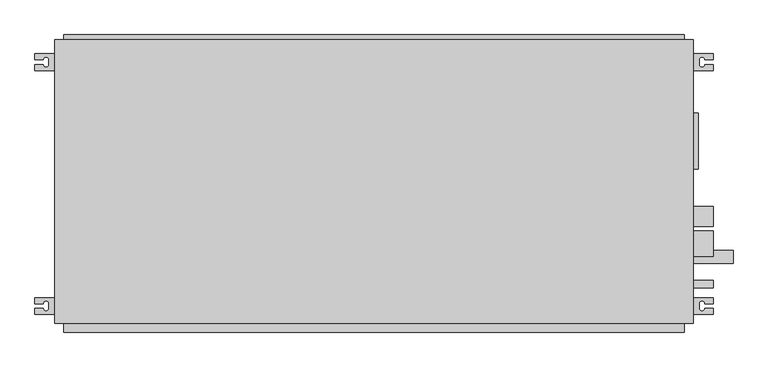
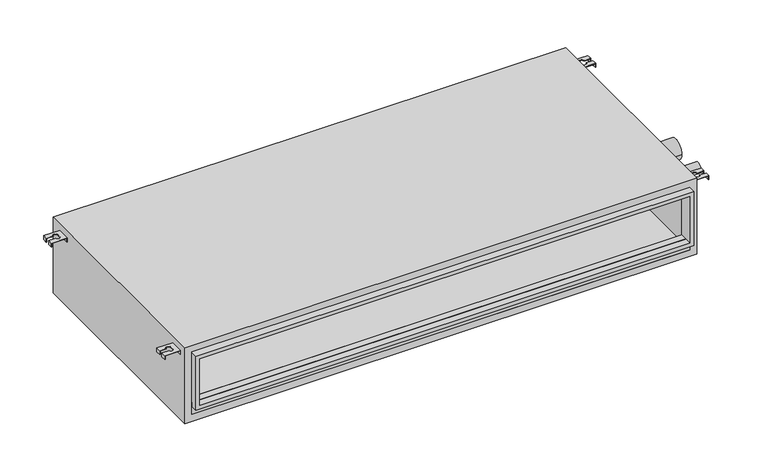
"""IFC4 building model written with IfcOpenShell, lengths in millimetres: proxy geometry, PEFY-P-NMAU-E_Medium_Static_Ducted : PEFY-P54NMAU-E."""

from ifc_helpers import new_model, si_unit, point, frame, frame_2d, origin, place, context, project, spatial, polyline, circle_curve, trimmed, segment, composite_curve, outline, extrude, source, transform, mapped, element, save
from ifc_brep_helpers import plane_surface, revolved_surface, advanced_brep


def mechanical_equipment_8a2286fb(model_context):
    return source(origin(), model_context, "Body", "SolidModel", [
        advanced_brep(
        [(-860.118493, -231.05, 249.2375), (-860.118493, -246.05, 249.2375), (-839.112243, -246.05, 249.2375), (-825.112243, -246.05, 249.2375), (-825.112243, -258.05, 249.2375), (-839.112243, -258.05, 249.2375), (-860.118493, -258.05, 249.2375), (-860.118493, -273.05, 249.2375), (-810.112243, -273.05, 249.2375), (-810.112243, -231.05, 249.2375), (-860.118493, -231.05, 236.4972162), (-858.530493, -231.05, 236.4972162), (-858.530493, -246.05, 236.4972162), (-860.118493, -246.05, 236.4972162), (-858.530493, -273.05, 236.4972162), (-860.118493, -273.05, 236.4972162), (-860.118493, -258.05, 236.4972162), (-858.530493, -258.05, 236.4972162), (-810.112243, -231.05, 236.4972162), (-810.112243, -273.05, 236.4972162), (-811.700243, -273.05, 236.4972162), (-811.700243, -231.05, 236.4972162), (-858.530493, -246.05, 247.65), (-839.112243, -246.05, 247.65), (-858.530493, -231.05, 247.65), (-811.700243, -231.05, 247.65), (-858.530493, -258.05, 247.65), (-858.530493, -273.05, 247.65), (-839.112243, -258.05, 247.65), (-811.700243, -273.05, 247.65), (-825.112243, -258.05, 247.65), (-825.112243, -246.05, 247.65)],
        [
            (0, 1),
            (1, 2),
            (2, 3, circle_curve(frame((-832.112243, -246.05, 249.2375), z_axis=(0.0, 0.0, -1.0), x_axis=(1.0, 0.0, 0.0)), 7.0)),
            (3, 4),
            (4, 5, circle_curve(frame((-832.112243, -258.05, 249.2375), z_axis=(0.0, 0.0, -1.0), x_axis=(1.0, 0.0, 0.0)), 7.0)),
            (5, 6),
            (6, 7),
            (7, 8),
            (8, 9),
            (9, 0),
            (10, 11),
            (11, 12),
            (12, 13),
            (13, 10),
            (14, 15),
            (15, 16),
            (16, 17),
            (17, 14),
            (18, 19),
            (19, 20),
            (20, 21),
            (21, 18),
            (13, 1),
            (0, 10),
            (12, 22),
            (22, 23),
            (23, 2),
            (11, 24),
            (24, 22),
            (9, 18),
            (21, 25),
            (25, 24),
            (17, 26),
            (26, 27),
            (27, 14),
            (5, 28),
            (28, 26),
            (16, 6),
            (15, 7),
            (27, 29),
            (29, 20),
            (19, 8),
            (29, 25),
            (30, 31),
            (31, 23, circle_curve(frame((-832.112243, -246.05, 247.65), z_axis=(0.0, 0.0, 1.0), x_axis=(1.0, 0.0, 0.0)), 7.0)),
            (28, 30, circle_curve(frame((-832.112243, -258.05, 247.65), z_axis=(0.0, 0.0, 1.0), x_axis=(1.0, 0.0, 0.0)), 7.0)),
            (4, 30),
            (31, 3),
        ],
        [
            plane_surface(frame((-860.118493, -231.05, 249.2375), z_axis=(0.0, 0.0, 1.0), x_axis=(0.0, -1.0, 0.0))),
            plane_surface(frame((-860.118493, -231.05, 236.4972162), z_axis=(0.0, 0.0, -1.0), x_axis=(0.0, 1.0, 0.0))),
            plane_surface(frame((-860.118493, -231.05, 249.2375), z_axis=(-1.0, 0.0, 0.0), x_axis=(0.0, 0.0, -1.0))),
            plane_surface(frame((-860.118493, -246.05, 249.2375), z_axis=(0.0, -1.0, 0.0), x_axis=(0.0, 0.0, -1.0))),
            plane_surface(frame((-858.530493, -246.05, 249.2375), z_axis=(1.0, 0.0, 0.0), x_axis=(0.0, 0.0, -1.0))),
            plane_surface(frame((-858.530493, -231.05, 249.2375), z_axis=(0.0, 1.0, 0.0), x_axis=(0.0, 0.0, -1.0))),
            plane_surface(frame((-858.530493, -273.05, 249.2375), z_axis=(1.0, 0.0, 0.0), x_axis=(0.0, 0.0, -1.0))),
            plane_surface(frame((-858.530493, -258.05, 249.2375), z_axis=(0.0, 1.0, 0.0), x_axis=(0.0, 0.0, -1.0))),
            plane_surface(frame((-860.118493, -258.05, 249.2375), z_axis=(-1.0, 0.0, 0.0), x_axis=(0.0, 0.0, -1.0))),
            plane_surface(frame((-860.118493, -273.05, 249.2375), z_axis=(0.0, -1.0, 0.0), x_axis=(0.0, 0.0, -1.0))),
            plane_surface(frame((-811.700243, -231.05, 249.2375), z_axis=(-1.0, 0.0, 0.0), x_axis=(0.0, 0.0, -1.0))),
            plane_surface(frame((-810.112243, -273.05, 249.2375), z_axis=(1.0, 0.0, 0.0), x_axis=(0.0, 0.0, -1.0))),
            plane_surface(frame((-825.112243, -258.05, 247.65), z_axis=(0.0, 0.0, -1.0), x_axis=(0.0, 1.0, 0.0))),
            revolved_surface(polyline([(-825.112243, -258.05, 247.65), (-825.112243, -258.05, 249.2375)]), (-832.112243, -258.05, 247.65), (0.0, 0.0, -1.0)),
            revolved_surface(polyline([(-825.112243, -246.05, 247.65), (-825.112243, -246.05, 249.2375)]), (-832.112243, -246.05, 247.65), (0.0, 0.0, -1.0)),
            plane_surface(frame((-825.112243, -246.05, 249.2375), z_axis=(-1.0, 0.0, 0.0), x_axis=(0.0, 0.0, -1.0))),
        ],
        [
            (0, [[1, 2, 3, 4, 5, 6, 7, 8, 9, 10]]),
            (1, [[11, 12, 13, 14]]),
            (1, [[15, 16, 17, 18]]),
            (1, [[19, 20, 21, 22]]),
            (2, [[23, -1, 24, -14]]),
            (3, [[-2, -23, -13, 25, 26, 27]]),
            (4, [[-12, 28, 29, -25]]),
            (5, [[-10, 30, -22, 31, 32, -28, -11, -24]]),
            (6, [[-18, 33, 34, 35]]),
            (7, [[-6, 36, 37, -33, -17, 38]]),
            (8, [[39, -7, -38, -16]]),
            (9, [[-8, -39, -15, -35, 40, 41, -20, 42]]),
            (10, [[-21, -41, 43, -31]]),
            (11, [[-30, -9, -42, -19]]),
            (12, [[44, 45, -26, -29, -32, -43, -40, -34, -37, 46]]),
            (13, [[-5, 47, -46, -36]]),
            (14, [[-3, -27, -45, 48]]),
            (15, [[-4, -48, -44, -47]]),
        ],
    ),
        advanced_brep(
        [(840.094007, -231.05, 249.2375), (790.087757, -231.05, 249.2375), (790.087757, -273.05, 249.2375), (840.094007, -273.05, 249.2375), (840.094007, -258.05, 249.2375), (819.087757, -258.05, 249.2375), (805.087757, -258.05, 249.2375), (805.087757, -246.05, 249.2375), (819.087757, -246.05, 249.2375), (840.094007, -246.05, 249.2375), (840.094007, -231.05, 236.4972162), (840.094007, -246.05, 236.4972162), (838.506007, -246.05, 236.4972162), (838.506007, -231.05, 236.4972162), (838.506007, -273.05, 236.4972162), (838.506007, -258.05, 236.4972162), (840.094007, -258.05, 236.4972162), (840.094007, -273.05, 236.4972162), (790.087757, -231.05, 236.4972162), (791.675757, -231.05, 236.4972162), (791.675757, -273.05, 236.4972162), (790.087757, -273.05, 236.4972162), (819.087757, -246.05, 247.65), (838.506007, -246.05, 247.65), (838.506007, -231.05, 247.65), (791.675757, -231.05, 247.65), (838.506007, -273.05, 247.65), (838.506007, -258.05, 247.65), (819.087757, -258.05, 247.65), (791.675757, -273.05, 247.65), (805.087757, -258.05, 247.65), (805.087757, -246.05, 247.65)],
        [
            (0, 1),
            (1, 2),
            (2, 3),
            (3, 4),
            (4, 5),
            (5, 6, circle_curve(frame((812.087757, -258.05, 249.2375), z_axis=(0.0, 0.0, -1.0), x_axis=(-1.0, 0.0, 0.0)), 7.0)),
            (6, 7),
            (7, 8, circle_curve(frame((812.087757, -246.05, 249.2375), z_axis=(0.0, 0.0, -1.0), x_axis=(-1.0, 0.0, 0.0)), 7.0)),
            (8, 9),
            (9, 0),
            (10, 11),
            (11, 12),
            (12, 13),
            (13, 10),
            (14, 15),
            (15, 16),
            (16, 17),
            (17, 14),
            (18, 19),
            (19, 20),
            (20, 21),
            (21, 18),
            (10, 0),
            (9, 11),
            (8, 22),
            (22, 23),
            (23, 12),
            (23, 24),
            (24, 13),
            (24, 25),
            (25, 19),
            (18, 1),
            (14, 26),
            (26, 27),
            (27, 15),
            (4, 16),
            (27, 28),
            (28, 5),
            (3, 17),
            (2, 21),
            (20, 29),
            (29, 26),
            (25, 29),
            (30, 28, circle_curve(frame((812.087757, -258.05, 247.65), z_axis=(0.0, 0.0, 1.0), x_axis=(-1.0, 0.0, 0.0)), 7.0)),
            (22, 31, circle_curve(frame((812.087757, -246.05, 247.65), z_axis=(0.0, 0.0, 1.0), x_axis=(-1.0, 0.0, 0.0)), 7.0)),
            (31, 30),
            (30, 6),
            (7, 31),
        ],
        [
            plane_surface(frame((840.094007, -231.05, 249.2375), z_axis=(0.0, 0.0, 1.0), x_axis=(0.0, -1.0, 0.0))),
            plane_surface(frame((840.094007, -231.05, 236.4972162), z_axis=(0.0, 0.0, -1.0), x_axis=(0.0, 1.0, 0.0))),
            plane_surface(frame((840.094007, -231.05, 249.2375), z_axis=(1.0, 0.0, 0.0), x_axis=(0.0, 0.0, -1.0))),
            plane_surface(frame((840.094007, -246.05, 249.2375), z_axis=(0.0, -1.0, 0.0), x_axis=(0.0, 0.0, -1.0))),
            plane_surface(frame((838.506007, -246.05, 249.2375), z_axis=(-1.0, 0.0, 0.0), x_axis=(0.0, 0.0, -1.0))),
            plane_surface(frame((838.506007, -231.05, 249.2375), z_axis=(0.0, 1.0, 0.0), x_axis=(0.0, 0.0, -1.0))),
            plane_surface(frame((838.506007, -273.05, 249.2375), z_axis=(-1.0, 0.0, 0.0), x_axis=(0.0, 0.0, -1.0))),
            plane_surface(frame((838.506007, -258.05, 249.2375), z_axis=(0.0, 1.0, 0.0), x_axis=(0.0, 0.0, -1.0))),
            plane_surface(frame((840.094007, -258.05, 249.2375), z_axis=(1.0, 0.0, 0.0), x_axis=(0.0, 0.0, -1.0))),
            plane_surface(frame((840.094007, -273.05, 249.2375), z_axis=(0.0, -1.0, 0.0), x_axis=(0.0, 0.0, -1.0))),
            plane_surface(frame((791.675757, -231.05, 249.2375), z_axis=(1.0, 0.0, 0.0), x_axis=(0.0, 0.0, -1.0))),
            plane_surface(frame((790.087757, -273.05, 249.2375), z_axis=(-1.0, 0.0, 0.0), x_axis=(0.0, 0.0, -1.0))),
            plane_surface(frame((805.087757, -258.05, 247.65), z_axis=(0.0, 0.0, -1.0), x_axis=(0.0, 1.0, 0.0))),
            revolved_surface(polyline([(805.087757, -258.05, 247.65), (805.087757, -258.05, 249.2375)]), (812.087757, -258.05, 247.65), (0.0, 0.0, -1.0)),
            revolved_surface(polyline([(805.087757, -246.05, 247.65), (805.087757, -246.05, 249.2375)]), (812.087757, -246.05, 247.65), (0.0, 0.0, -1.0)),
            plane_surface(frame((805.087757, -246.05, 249.2375), z_axis=(1.0, 0.0, 0.0), x_axis=(0.0, 0.0, -1.0))),
        ],
        [
            (0, [[1, 2, 3, 4, 5, 6, 7, 8, 9, 10]]),
            (1, [[11, 12, 13, 14]]),
            (1, [[15, 16, 17, 18]]),
            (1, [[19, 20, 21, 22]]),
            (2, [[-11, 23, -10, 24]]),
            (3, [[25, 26, 27, -12, -24, -9]]),
            (4, [[-27, 28, 29, -13]]),
            (5, [[-23, -14, -29, 30, 31, -19, 32, -1]]),
            (6, [[33, 34, 35, -15]]),
            (7, [[36, -16, -35, 37, 38, -5]]),
            (8, [[-17, -36, -4, 39]]),
            (9, [[40, -21, 41, 42, -33, -18, -39, -3]]),
            (10, [[-31, 43, -41, -20]]),
            (11, [[-22, -40, -2, -32]]),
            (12, [[44, -37, -34, -42, -43, -30, -28, -26, 45, 46]]),
            (13, [[-38, -44, 47, -6]]),
            (14, [[48, -45, -25, -8]]),
            (15, [[-47, -46, -48, -7]]),
        ],
    ),
        advanced_brep(
        [(-860.118493, 339.0, 249.2375), (-810.112243, 339.0, 249.2375), (-810.112243, 381.0, 249.2375), (-860.118493, 381.0, 249.2375), (-860.118493, 366.0, 249.2375), (-839.112243, 366.0, 249.2375), (-825.112243, 366.0, 249.2375), (-825.112243, 354.0, 249.2375), (-839.112243, 354.0, 249.2375), (-860.118493, 354.0, 249.2375), (-860.118493, 339.0, 236.4972162), (-860.118493, 354.0, 236.4972162), (-858.530493, 354.0, 236.4972162), (-858.530493, 339.0, 236.4972162), (-858.530493, 381.0, 236.4972162), (-858.530493, 366.0, 236.4972162), (-860.118493, 366.0, 236.4972162), (-860.118493, 381.0, 236.4972162), (-810.112243, 339.0, 236.4972162), (-811.700243, 339.0, 236.4972162), (-811.700243, 381.0, 236.4972162), (-810.112243, 381.0, 236.4972162), (-839.112243, 354.0, 247.65), (-858.530493, 354.0, 247.65), (-858.530493, 339.0, 247.65), (-811.700243, 339.0, 247.65), (-858.530493, 381.0, 247.65), (-858.530493, 366.0, 247.65), (-839.112243, 366.0, 247.65), (-811.700243, 381.0, 247.65), (-825.112243, 366.0, 247.65), (-825.112243, 354.0, 247.65)],
        [
            (0, 1),
            (1, 2),
            (2, 3),
            (3, 4),
            (4, 5),
            (5, 6, circle_curve(frame((-832.112243, 366.0, 249.2375), z_axis=(0.0, 0.0, -1.0), x_axis=(1.0, 0.0, 0.0)), 7.0)),
            (6, 7),
            (7, 8, circle_curve(frame((-832.112243, 354.0, 249.2375), z_axis=(0.0, 0.0, -1.0), x_axis=(1.0, 0.0, 0.0)), 7.0)),
            (8, 9),
            (9, 0),
            (10, 11),
            (11, 12),
            (12, 13),
            (13, 10),
            (14, 15),
            (15, 16),
            (16, 17),
            (17, 14),
            (18, 19),
            (19, 20),
            (20, 21),
            (21, 18),
            (10, 0),
            (9, 11),
            (8, 22),
            (22, 23),
            (23, 12),
            (23, 24),
            (24, 13),
            (24, 25),
            (25, 19),
            (18, 1),
            (14, 26),
            (26, 27),
            (27, 15),
            (4, 16),
            (27, 28),
            (28, 5),
            (3, 17),
            (2, 21),
            (20, 29),
            (29, 26),
            (25, 29),
            (30, 28, circle_curve(frame((-832.112243, 366.0, 247.65), z_axis=(0.0, 0.0, 1.0), x_axis=(1.0, 0.0, 0.0)), 7.0)),
            (22, 31, circle_curve(frame((-832.112243, 354.0, 247.65), z_axis=(0.0, 0.0, 1.0), x_axis=(1.0, 0.0, 0.0)), 7.0)),
            (31, 30),
            (30, 6),
            (7, 31),
        ],
        [
            plane_surface(frame((-860.118493, 339.0, 249.2375), z_axis=(0.0, 0.0, 1.0), x_axis=(0.0, 1.0, 0.0))),
            plane_surface(frame((-860.118493, 339.0, 236.4972162), z_axis=(0.0, 0.0, -1.0), x_axis=(0.0, -1.0, 0.0))),
            plane_surface(frame((-860.118493, 339.0, 249.2375), z_axis=(-1.0, 0.0, 0.0), x_axis=(0.0, 0.0, -1.0))),
            plane_surface(frame((-860.118493, 354.0, 249.2375), z_axis=(0.0, 1.0, 0.0), x_axis=(0.0, 0.0, -1.0))),
            plane_surface(frame((-858.530493, 354.0, 249.2375), z_axis=(1.0, 0.0, 0.0), x_axis=(0.0, 0.0, -1.0))),
            plane_surface(frame((-858.530493, 339.0, 249.2375), z_axis=(0.0, -1.0, 0.0), x_axis=(0.0, 0.0, -1.0))),
            plane_surface(frame((-858.530493, 381.0, 249.2375), z_axis=(1.0, 0.0, 0.0), x_axis=(0.0, 0.0, -1.0))),
            plane_surface(frame((-858.530493, 366.0, 249.2375), z_axis=(0.0, -1.0, 0.0), x_axis=(0.0, 0.0, -1.0))),
            plane_surface(frame((-860.118493, 366.0, 249.2375), z_axis=(-1.0, 0.0, 0.0), x_axis=(0.0, 0.0, -1.0))),
            plane_surface(frame((-860.118493, 381.0, 249.2375), z_axis=(0.0, 1.0, 0.0), x_axis=(0.0, 0.0, -1.0))),
            plane_surface(frame((-811.700243, 339.0, 249.2375), z_axis=(-1.0, 0.0, 0.0), x_axis=(0.0, 0.0, -1.0))),
            plane_surface(frame((-810.112243, 381.0, 249.2375), z_axis=(1.0, 0.0, 0.0), x_axis=(0.0, 0.0, -1.0))),
            plane_surface(frame((-825.112243, 366.0, 247.65), z_axis=(0.0, 0.0, -1.0), x_axis=(0.0, -1.0, 0.0))),
            revolved_surface(polyline([(-825.112243, 366.0, 247.65), (-825.112243, 366.0, 249.2375)]), (-832.112243, 366.0, 247.65), (0.0, 0.0, -1.0)),
            revolved_surface(polyline([(-825.112243, 354.0, 247.65), (-825.112243, 354.0, 249.2375)]), (-832.112243, 354.0, 247.65), (0.0, 0.0, -1.0)),
            plane_surface(frame((-825.112243, 354.0, 249.2375), z_axis=(-1.0, 0.0, 0.0), x_axis=(0.0, 0.0, -1.0))),
        ],
        [
            (0, [[1, 2, 3, 4, 5, 6, 7, 8, 9, 10]]),
            (1, [[11, 12, 13, 14]]),
            (1, [[15, 16, 17, 18]]),
            (1, [[19, 20, 21, 22]]),
            (2, [[-11, 23, -10, 24]]),
            (3, [[25, 26, 27, -12, -24, -9]]),
            (4, [[-27, 28, 29, -13]]),
            (5, [[-23, -14, -29, 30, 31, -19, 32, -1]]),
            (6, [[33, 34, 35, -15]]),
            (7, [[36, -16, -35, 37, 38, -5]]),
            (8, [[-17, -36, -4, 39]]),
            (9, [[40, -21, 41, 42, -33, -18, -39, -3]]),
            (10, [[-31, 43, -41, -20]]),
            (11, [[-22, -40, -2, -32]]),
            (12, [[44, -37, -34, -42, -43, -30, -28, -26, 45, 46]]),
            (13, [[-38, -44, 47, -6]]),
            (14, [[48, -45, -25, -8]]),
            (15, [[-47, -46, -48, -7]]),
        ],
    ),
        advanced_brep(
        [(840.094007, 339.0, 249.2375), (840.094007, 354.0, 249.2375), (819.087757, 354.0, 249.2375), (805.087757, 354.0, 249.2375), (805.087757, 366.0, 249.2375), (819.087757, 366.0, 249.2375), (840.094007, 366.0, 249.2375), (840.094007, 381.0, 249.2375), (790.087757, 381.0, 249.2375), (790.087757, 339.0, 249.2375), (840.094007, 339.0, 236.4972162), (838.506007, 339.0, 236.4972162), (838.506007, 354.0, 236.4972162), (840.094007, 354.0, 236.4972162), (838.506007, 381.0, 236.4972162), (840.094007, 381.0, 236.4972162), (840.094007, 366.0, 236.4972162), (838.506007, 366.0, 236.4972162), (790.087757, 339.0, 236.4972162), (790.087757, 381.0, 236.4972162), (791.675757, 381.0, 236.4972162), (791.675757, 339.0, 236.4972162), (838.506007, 354.0, 247.65), (819.087757, 354.0, 247.65), (838.506007, 339.0, 247.65), (791.675757, 339.0, 247.65), (838.506007, 366.0, 247.65), (838.506007, 381.0, 247.65), (819.087757, 366.0, 247.65), (791.675757, 381.0, 247.65), (805.087757, 366.0, 247.65), (805.087757, 354.0, 247.65)],
        [
            (0, 1),
            (1, 2),
            (2, 3, circle_curve(frame((812.087757, 354.0, 249.2375), z_axis=(0.0, 0.0, -1.0), x_axis=(-1.0, 0.0, 0.0)), 7.0)),
            (3, 4),
            (4, 5, circle_curve(frame((812.087757, 366.0, 249.2375), z_axis=(0.0, 0.0, -1.0), x_axis=(-1.0, 0.0, 0.0)), 7.0)),
            (5, 6),
            (6, 7),
            (7, 8),
            (8, 9),
            (9, 0),
            (10, 11),
            (11, 12),
            (12, 13),
            (13, 10),
            (14, 15),
            (15, 16),
            (16, 17),
            (17, 14),
            (18, 19),
            (19, 20),
            (20, 21),
            (21, 18),
            (13, 1),
            (0, 10),
            (12, 22),
            (22, 23),
            (23, 2),
            (11, 24),
            (24, 22),
            (9, 18),
            (21, 25),
            (25, 24),
            (17, 26),
            (26, 27),
            (27, 14),
            (5, 28),
            (28, 26),
            (16, 6),
            (15, 7),
            (27, 29),
            (29, 20),
            (19, 8),
            (29, 25),
            (30, 31),
            (31, 23, circle_curve(frame((812.087757, 354.0, 247.65), z_axis=(0.0, 0.0, 1.0), x_axis=(-1.0, 0.0, 0.0)), 7.0)),
            (28, 30, circle_curve(frame((812.087757, 366.0, 247.65), z_axis=(0.0, 0.0, 1.0), x_axis=(-1.0, 0.0, 0.0)), 7.0)),
            (4, 30),
            (31, 3),
        ],
        [
            plane_surface(frame((840.094007, 339.0, 249.2375), z_axis=(0.0, 0.0, 1.0), x_axis=(0.0, 1.0, 0.0))),
            plane_surface(frame((840.094007, 339.0, 236.4972162), z_axis=(0.0, 0.0, -1.0), x_axis=(0.0, -1.0, 0.0))),
            plane_surface(frame((840.094007, 339.0, 249.2375), z_axis=(1.0, 0.0, 0.0), x_axis=(0.0, 0.0, -1.0))),
            plane_surface(frame((840.094007, 354.0, 249.2375), z_axis=(0.0, 1.0, 0.0), x_axis=(0.0, 0.0, -1.0))),
            plane_surface(frame((838.506007, 354.0, 249.2375), z_axis=(-1.0, 0.0, 0.0), x_axis=(0.0, 0.0, -1.0))),
            plane_surface(frame((838.506007, 339.0, 249.2375), z_axis=(0.0, -1.0, 0.0), x_axis=(0.0, 0.0, -1.0))),
            plane_surface(frame((838.506007, 381.0, 249.2375), z_axis=(-1.0, 0.0, 0.0), x_axis=(0.0, 0.0, -1.0))),
            plane_surface(frame((838.506007, 366.0, 249.2375), z_axis=(0.0, -1.0, 0.0), x_axis=(0.0, 0.0, -1.0))),
            plane_surface(frame((840.094007, 366.0, 249.2375), z_axis=(1.0, 0.0, 0.0), x_axis=(0.0, 0.0, -1.0))),
            plane_surface(frame((840.094007, 381.0, 249.2375), z_axis=(0.0, 1.0, 0.0), x_axis=(0.0, 0.0, -1.0))),
            plane_surface(frame((791.675757, 339.0, 249.2375), z_axis=(1.0, 0.0, 0.0), x_axis=(0.0, 0.0, -1.0))),
            plane_surface(frame((790.087757, 381.0, 249.2375), z_axis=(-1.0, 0.0, 0.0), x_axis=(0.0, 0.0, -1.0))),
            plane_surface(frame((805.087757, 366.0, 247.65), z_axis=(0.0, 0.0, -1.0), x_axis=(0.0, -1.0, 0.0))),
            revolved_surface(polyline([(805.087757, 366.0, 247.65), (805.087757, 366.0, 249.2375)]), (812.087757, 366.0, 247.65), (0.0, 0.0, -1.0)),
            revolved_surface(polyline([(805.087757, 354.0, 247.65), (805.087757, 354.0, 249.2375)]), (812.087757, 354.0, 247.65), (0.0, 0.0, -1.0)),
            plane_surface(frame((805.087757, 354.0, 249.2375), z_axis=(1.0, 0.0, 0.0), x_axis=(0.0, 0.0, -1.0))),
        ],
        [
            (0, [[1, 2, 3, 4, 5, 6, 7, 8, 9, 10]]),
            (1, [[11, 12, 13, 14]]),
            (1, [[15, 16, 17, 18]]),
            (1, [[19, 20, 21, 22]]),
            (2, [[23, -1, 24, -14]]),
            (3, [[-2, -23, -13, 25, 26, 27]]),
            (4, [[-12, 28, 29, -25]]),
            (5, [[-10, 30, -22, 31, 32, -28, -11, -24]]),
            (6, [[-18, 33, 34, 35]]),
            (7, [[-6, 36, 37, -33, -17, 38]]),
            (8, [[39, -7, -38, -16]]),
            (9, [[-8, -39, -15, -35, 40, 41, -20, 42]]),
            (10, [[-21, -41, 43, -31]]),
            (11, [[-30, -9, -42, -19]]),
            (12, [[44, 45, -26, -29, -32, -43, -40, -34, -37, 46]]),
            (13, [[-5, 47, -46, -36]]),
            (14, [[-3, -27, -45, 48]]),
            (15, [[-4, -48, -44, -47]]),
        ],
    ),
        extrude(outline(polyline([(767.862757, -295.275), (-787.887243, -295.275), (-787.887243, -273.05), (767.862757, -273.05), (767.862757, -295.275)])), frame((0.0, 0.0, 42.8625), z_axis=(0.0, 0.0, 1.0), x_axis=(1.0, 0.0, 0.0)), (0.0, 0.0, 1.0), 39.6875),
        extrude(outline(polyline([(249.2375, 767.862757), (249.2375, -787.887243), (69.85, -787.887243), (69.85, 767.862757), (249.2375, 767.862757)]), holes=[polyline([(82.55, 755.162757), (82.55, -775.187243), (236.5375, -775.187243), (236.5375, 755.162757), (82.55, 755.162757)])]), frame((0.0, -317.5, 0.0), z_axis=(0.0, 1.0, 0.0), x_axis=(0.0, 0.0, 1.0)), (0.0, 0.0, 1.0), 44.45),
        extrude(outline(polyline([(767.862757, 415.925), (-787.887243, 415.925), (-787.887243, 428.625), (767.862757, 428.625), (767.862757, 415.925)])), frame((0.0, 0.0, 42.8625), z_axis=(0.0, 0.0, 1.0), x_axis=(1.0, 0.0, 0.0)), (0.0, 0.0, 1.0), 206.375),
        extrude(outline(polyline([(271.4625, 790.087757), (271.4625, -810.112243), (20.6375, -810.112243), (20.6375, 790.087757), (271.4625, 790.087757)]), holes=[polyline([(42.8625, -787.887243), (249.2375, -787.887243), (249.2375, 767.862757), (42.8625, 767.862757), (42.8625, -787.887243)])]), frame((0.0, -295.275, 0.0), z_axis=(0.0, 1.0, 0.0), x_axis=(0.0, 0.0, 1.0)), (0.0, 0.0, 1.0), 711.2),
        extrude(outline(composite_curve([segment(trimmed(circle_curve(frame_2d((-26.9875, 109.5375)), 25.4), [point((-1.5875, 109.5375))], [point((-52.3875, 109.5375))], False, "CARTESIAN"), True, "CONTINUOUS"), segment(trimmed(circle_curve(frame_2d((-26.9875, 109.5375)), 25.4), [point((-52.3875, 109.5375))], [point((-1.5875, 109.5375))], False, "CARTESIAN"), True, "CONTINUOUS")], self_intersect=False)), frame((790.087757, 0.0, 0.0), z_axis=(1.0, 0.0, 0.0), x_axis=(0.0, 1.0, 0.0)), (0.0, 0.0, 1.0), 50.00625),
        extrude(outline(composite_curve([segment(trimmed(circle_curve(frame_2d((-128.5875, 171.45)), 15.875), [point((-112.7125, 171.45))], [point((-144.4625, 171.45))], False, "CARTESIAN"), True, "CONTINUOUS"), segment(trimmed(circle_curve(frame_2d((-128.5875, 171.45)), 15.875), [point((-144.4625, 171.45))], [point((-112.7125, 171.45))], False, "CARTESIAN"), True, "CONTINUOUS")], self_intersect=False)), frame((790.087757, 0.0, 0.0), z_axis=(1.0, 0.0, 0.0), x_axis=(0.0, 1.0, 0.0)), (0.0, 0.0, 1.0), 100.0125),
        extrude(outline(composite_curve([segment(trimmed(circle_curve(frame_2d((-95.25, 230.1875)), 31.75), [point((-63.5, 230.1875))], [point((-127.0, 230.1875))], False, "CARTESIAN"), True, "CONTINUOUS"), segment(trimmed(circle_curve(frame_2d((-95.25, 230.1875)), 31.75), [point((-127.0, 230.1875))], [point((-63.5, 230.1875))], False, "CARTESIAN"), True, "CONTINUOUS")], self_intersect=False)), frame((790.087757, 0.0, 0.0), z_axis=(1.0, 0.0, 0.0), x_axis=(0.0, 1.0, 0.0)), (0.0, 0.0, 1.0), 50.00625),
        extrude(outline(composite_curve([segment(trimmed(circle_curve(frame_2d((-196.85, 104.775)), 9.525), [point((-187.325, 104.775))], [point((-206.375, 104.775))], False, "CARTESIAN"), True, "CONTINUOUS"), segment(trimmed(circle_curve(frame_2d((-196.85, 104.775)), 9.525), [point((-206.375, 104.775))], [point((-187.325, 104.775))], False, "CARTESIAN"), True, "CONTINUOUS")], self_intersect=False)), frame((790.087757, 0.0, 0.0), z_axis=(1.0, 0.0, 0.0), x_axis=(0.0, 1.0, 0.0)), (0.0, 0.0, 1.0), 50.00625),
        extrude(outline(polyline([(802.787757, 231.84375), (802.787757, 92.14375), (790.087757, 92.14375), (790.087757, 231.84375), (802.787757, 231.84375)])), frame((0.0, 0.0, 42.8625), z_axis=(0.0, 0.0, 1.0), x_axis=(1.0, 0.0, 0.0)), (0.0, 0.0, 1.0), 187.325),
    ])


if __name__ == "__main__":
    model = new_model("IFC4")
    model_context = context("Model", 3, world=origin())
    ifc_project = project(units=[si_unit("LENGTHUNIT", "METRE", prefix="MILLI")], contexts=[model_context])
    site = spatial("IfcSite", under=ifc_project)
    building = spatial("IfcBuilding", under=site)
    placement = place(None, origin())
    mechanical_equipment_shape = mechanical_equipment_8a2286fb(model_context)
    element("IfcBuildingElementProxy", 1, Name="PEFY-P-NMAU-E_Medium_Static_Ducted : PEFY-P54NMAU-E", ObjectType="PEFY-P-NMAU-E_Medium_Static_Ducted : PEFY-P54NMAU-E", at=placement, inside=building, context=model_context, shape_type="MappedRepresentation", body=[
        mapped(mechanical_equipment_shape, transform((0.0, 0.0, 0.0), x_axis=(1.0, 0.0, 0.0), y_axis=(0.0, 1.0, 0.0), z_axis=(0.0, 0.0, 1.0))),
    ])
    save(model, "model.ifc")

# Revit data of these elements
# Type "PEFY-P-NMAU-E_Medium_Static_Ducted : PEFY-P54NMAU-E"
#   Wiring (Min.size of wire) = "1/8"
#   Wiring (Amperage of wire breaker) = "15 A"
#   Voltage Options = "208/230 VAC"
#   Unit Weight (LBS) = "102"
#   Temperature set range Remote controller Heating = "63 to 83 F"
#   Temperature set range Remote controller Cooling = "67 to 86 F"
#   Subcategory = "HVAC"
#   Specification URL = ""
#   Sound Pressure Levels (dB(A)) = "26,28,29"
#   SmartBIM Object Created By = "Reed Construction Data"
#   Single Phase = "X"
#   Refrigerant control device = "LEV"
#   Protection devices = "Fuse"
#   Power input Heating = "0.34 kW"
#   Power input Cooling = "0.36 kW"
#   Moter Type = "DC blushless motor"
#   Moter Output = "0.085 kW"
#   Model = "PEFY-P54NMAU-E"
#   Manufacturer URL = ""
#   Manufacturer = "Mitsubishi Electric"
#   Insulation material = "EPS, Polyethylene foam, Urethane foam"
#   Installation URL = ""
#   Heating Capacity (kcal/h) = "15,100"
#   Heating Capacity (kW) = "17.6"
#   Heat exchanger = "Cross fin(Aluminium fin and copper tube)"
#   Frequency = "60 Hz"
#   Fan Type x Quantity = "Sirocco fan x 1"
#   E.S.P(mmH2O) = "3.6,5.1,7.1,10.2,15.3"
#   E.S.P(Pa) = "35,50,70,100,150"
#   E.S.P(In. W.G.) = "0.14,0.20,0.28,0.40,0.60"
#   Driving mechanism = "Direct-driven by motor"
#   Current Heating = "2.13 A"
#   Current Cooling = "2.24 A"
#   Cooling Capacity (kcal/h) = "13,600"
#   Cooling Capacity (kW) = "15.8"
#   Connectable outdoor unit = "R410A,R22 CITY MULTI"
#   Assembly Code = "D3050200"
#   Airflow rate(Low-Mid-High) (m3/min) = "6.0,7.5,8.5"
#   Airflow rate(Low-Mid-High) (cfm) = "212,265,300"
#   Airflow rate(Low-Mid-High) (L/s) = "100,125,142"
#   Air Filter = "PP Honeycomb fabric"
#   95 CSI = "15760"
#   04 CSI = "23 82 19"
#   Width = 1600.2 mm
#   Voltage = 208 V
#   Unit Supply Airflow [instance default] = 0 CFM
#   Unit Return Airflow [instance default] = 0 CFM
#   SmartBIM Object Version = 3
#   Refrigerant Pipe Liquid = 9.525 mm
#   Refrigerant Pipe Gas = 15.875 mm
#   Refirigerant Pipe diameter (Liquid) = 9.525 mm
#   Refirigerant Pipe diameter (Gas) = 15.875 mm
#   Phase = 1
#   Nominal Heating Capacity = 60000.0 Btu/h
#   Nominal Cooling Capacity = 54000.0 Btu/h
#   Minimum Circuit Current = 3.31 A
#   Maximum Overcurrent Protection = 15 A
#   Hertz = 60
#   Height = 250.825 mm
#   Drain piping diameter = 31.75 mm
#   Drain Pump = 25.4 mm
#   Depth = 733.425 mm
#   Default Elevation = 1219.2 mm
#   Back Air Inlet Width = 1555.75 mm
#   Back Air Inlet Height = 206.375 mm
#   Apparent Load = 0 VA
#   Air Outlet Width = 1555.75 mm
#   Air Outlet Height = 179.388 mm
#   Sound Pressure Levels @ Mid Airflow (dBA) = 41
#   Sound Pressure Levels @ Low Airflow (dBA) = 36
#   Sound Pressure Levels @ High Airflow (dBA) = 45
#   Number of Poles = 2
#   Unit = Metal - Steel Satin
#   Load Classification = Other
#   Back Air Inlet = Grille
# Element 1 (IfcBuildingElementProxy, "PEFY-P-NMAU-E_Medium_Static_Ducted : PEFY-P54NMAU-E")
#   Materials on its faces: "Metal - Steel Satin", "Grille"
# Materials
#   "Metal - Steel Satin": class "Metal", colour RGB 189 187 185, transparency 0
#   "Grille": class "Miscellaneous", colour RGB 0 0 0, transparency 0
